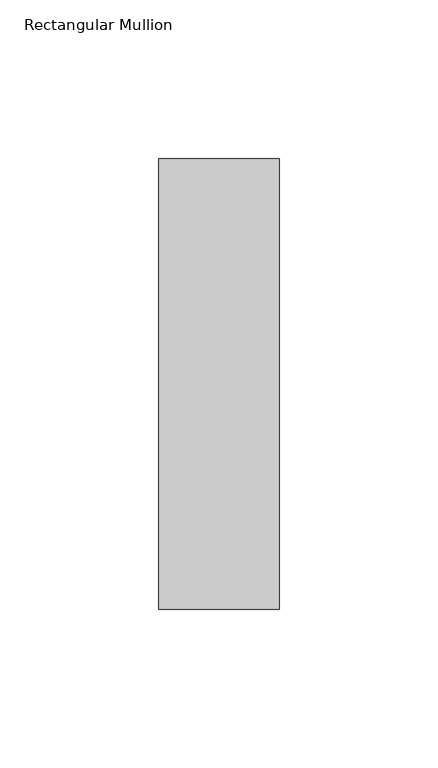
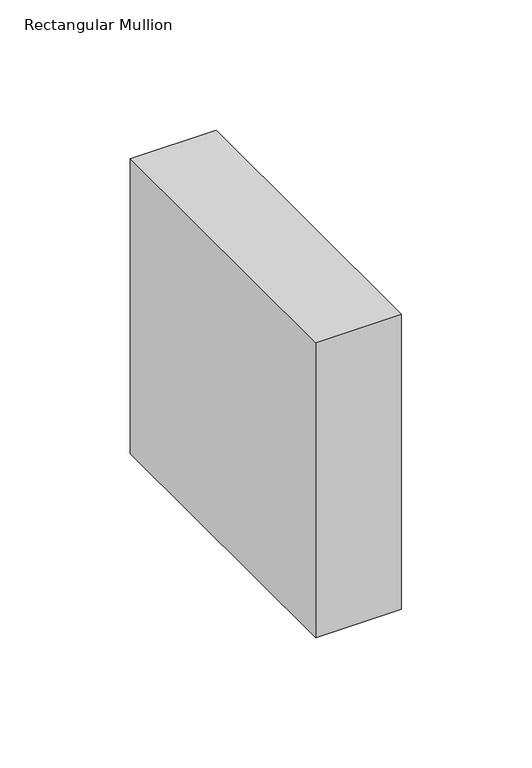
"""IFC4 building model written with IfcOpenShell, lengths in millimetres: member geometry, Rectangular Mullion : NLRS_21_CWM_hsb-regel 38x142_gen_rsf."""

from ifc_helpers import new_model, si_unit, frame, origin, place, context, project, spatial, polyline, outline, extrude, source, transform, mapped, element, save


def rectangular_mullion_ef8690d9(model_context):
    return source(origin(), model_context, "Body", "SweptSolid", [
        extrude(outline(polyline([(0.0, -71.0), (-38.0, -71.0), (-38.0, 71.0), (0.0, 71.0), (0.0, -71.0)])), frame((0.0, 0.0, -137.9999997), z_axis=(0.0, 0.0, 1.0), x_axis=(1.0, 0.0, 0.0)), (0.0, 0.0, 1.0), 137.9999997),
    ])


if __name__ == "__main__":
    model = new_model("IFC4")
    model_context = context("Model", 3, world=origin())
    ifc_project = project(units=[si_unit("LENGTHUNIT", "METRE", prefix="MILLI")], contexts=[model_context])
    site = spatial("IfcSite", under=ifc_project)
    building = spatial("IfcBuilding", under=site)
    placement = place(None, origin())
    rectangular_mullion_shape = rectangular_mullion_ef8690d9(model_context)
    element("IfcMember", 1, ObjectType="Rectangular Mullion : NLRS_21_CWM_hsb-regel 38x142_gen_rsf", at=placement, inside=building, context=model_context, shape_type="MappedRepresentation", body=[
        mapped(rectangular_mullion_shape, transform((0.0, 0.0, 0.0), x_axis=(1.0, 0.0, 0.0), y_axis=(0.0, 1.0, 0.0), z_axis=(0.0, 0.0, 1.0))),
    ])
    save(model, "model.ifc")

# Revit data of these elements
# Type "Rectangular Mullion : NLRS_21_CWM_hsb-regel 38x142_gen_rsf"
#   Export Type to IFC As = "IfcWall"
#   Type IfcGUID = "07M7mRoiH1CR8m_RSKIwpF"
#   Assembly Code = "21.10"
#   built-in parameter 1007322 = 0.465879 (stored number, unit not read)
#   built-in parameter 1007321 = 0.062336 (stored number, unit not read)
#   built-in parameter 1007320 = 0.062336 (stored number, unit not read)
# Element 1 (IfcMember, "Rectangular Mullion : NLRS_21_CWM_hsb-regel 38x142_gen_rsf")
#   Materials on its faces: "NLRS_i2_hout naaldhout vuren_gen_rsf"
# Materials
#   "NLRS_i2_hout naaldhout vuren_gen_rsf": class "I - Hout", colour RGB 234 199 147, transparency 0, Keynote = "i2", Manufacturer = "Revit Standards Foundation", URL = "www.revitstandards.org", Description = "hout vuren", Cost = 0
